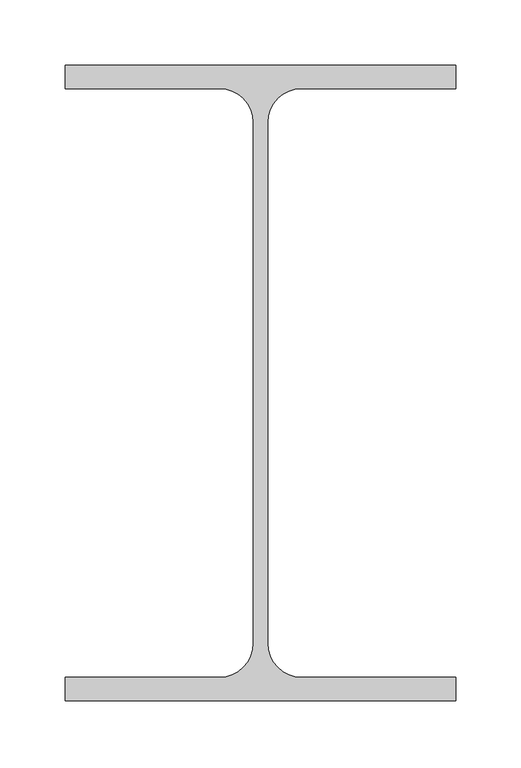
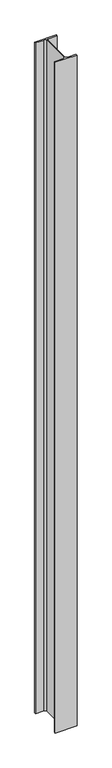
"""IFC4 building model written with IfcOpenShell, lengths in millimetres: column geometry, 0912_Steel Column_H_KSD3502 : H_SC_ASC_H-488x300x11x18."""

from ifc_helpers import new_model, si_unit, point, frame, frame_2d, origin, place, context, project, spatial, polyline, circle_curve, trimmed, segment, composite_curve, outline, extrude, source, transform, mapped, element, save


def column_bd22218f(model_context):
    return source(origin(), model_context, "Body", "SweptSolid", [
        extrude(outline(composite_curve([segment(polyline([(150.0, 244.0), (150.0, 226.0), (31.5, 226.0)]), True, "CONTINUOUS"), segment(trimmed(circle_curve(frame_2d((31.5, 200.0)), 26.0), [point((31.5, 226.0))], [point((5.5, 200.0))], True, "CARTESIAN"), True, "CONTINUOUS"), segment(polyline([(5.5, 200.0), (5.5, -200.0)]), True, "CONTINUOUS"), segment(trimmed(circle_curve(frame_2d((31.5, -200.0)), 26.0), [point((5.5, -200.0))], [point((31.5, -226.0))], True, "CARTESIAN"), True, "CONTINUOUS"), segment(polyline([(31.5, -226.0), (150.0, -226.0), (150.0, -244.0), (-150.0, -244.0), (-150.0, -226.0), (-31.5, -226.0)]), True, "CONTINUOUS"), segment(trimmed(circle_curve(frame_2d((-31.5, -200.0)), 26.0), [point((-31.5, -226.0))], [point((-5.5, -200.0))], True, "CARTESIAN"), True, "CONTINUOUS"), segment(polyline([(-5.5, -200.0), (-5.5, 200.0)]), True, "CONTINUOUS"), segment(trimmed(circle_curve(frame_2d((-31.5, 200.0)), 26.0), [point((-5.5, 200.0))], [point((-31.5, 226.0))], True, "CARTESIAN"), True, "CONTINUOUS"), segment(polyline([(-31.5, 226.0), (-150.0, 226.0), (-150.0, 244.0), (150.0, 244.0)]), True, "CONTINUOUS")], self_intersect=False)), frame((0.0, 0.0, 7538.9720055), z_axis=(0.0, 0.0, 1.0), x_axis=(1.0, 0.0, 0.0)), (0.0, 0.0, 1.0), 9761.0),
    ])


if __name__ == "__main__":
    model = new_model("IFC4")
    model_context = context("Model", 3, world=origin())
    ifc_project = project(units=[si_unit("LENGTHUNIT", "METRE", prefix="MILLI")], contexts=[model_context])
    site = spatial("IfcSite", under=ifc_project)
    building = spatial("IfcBuilding", under=site)
    placement = place(None, origin())
    column_shape = column_bd22218f(model_context)
    element("IfcColumn", 1, ObjectType="0912_Steel Column_H_KSD3502 : H_SC_ASC_H-488x300x11x18", at=placement, inside=building, context=model_context, shape_type="MappedRepresentation", body=[
        mapped(column_shape, transform((0.0, 0.0, 0.0), x_axis=(1.0, 0.0, 0.0), y_axis=(0.0, 1.0, 0.0), z_axis=(0.0, 0.0, 1.0))),
    ])
    save(model, "model.ifc")

# Revit data of these elements
# Type "0912_Steel Column_H_KSD3502 : H_SC_ASC_H-488x300x11x18"
#   H_WM Code_1 = "S01AA002-00001 | Main Steel Structure Fabrication Work | Shelter/Building | Medium Steel - Standard (90KG/M>Weight≥30KG/M) | Material: (   )"
#   H_WM Code_2 = "S03AA028-00001 | Main Steel Structure Erection Work | Shelter/Building | Medium Steel (90KG/M>Weight≥30KG/M) | Material: (   )"
#   H_WM Code_3 = "S01AA010-00001 | Main Steel Structure Fabrication Work | Shelter/Building | Steel Painting/Coating | for Non-Fireproofed Steel Surface, Surface Preparation, Primer, Second & Final Coat | Material: (   )"
#   H_Q'ty Cal Type Tag = "SC-Q2"
#   Width = 30.0 cm
#   Web Thickness = 1.1 cm
#   Web Fillet = 2.6 cm
#   Warping Constant = 4473230.0 cm⁶
#   Torsional Moment of Inertia = 137.492 cm⁴
#   Section Area = 163.5 cm²
#   Plastic Modulus weak axis = 830.0 cm³
#   Plastic Modulus strong axis = 3230.0 cm³
#   Perimeter = 2.11 m²/m
#   Nominal Weight = 128.00 kgf/m
#   Moment of Inertia weak axis = 8110.00 cm⁴
#   Moment of Inertia strong axis = 71000.00 cm⁴
#   Height = 48.8 cm
#   Flange Thickness = 1.8 cm
#   Elastic Modulus weak axis = 541.0 cm³
#   Elastic Modulus strong axis = 2910.0 cm³
#   Centroid Vertical = 24.4 cm
#   Centroid Horizontal = 15.0 cm
#   Structural Material [instance default] = Steel, 45-345
#   Section Name Key = ""
#   Bolt Spacing = 0
#   Assembly Code = ""
# Element 1 (IfcColumn, "0912_Steel Column_H_KSD3502 : H_SC_ASC_H-488x300x11x18")
#   Structural Material = none
# Materials
#   "Steel, 45-345": class "Metal", colour RGB 189 187 185, transparency 0, Description = "Steel 345 MPa", Cost = 0
